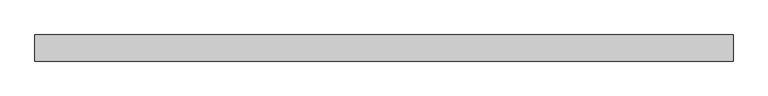
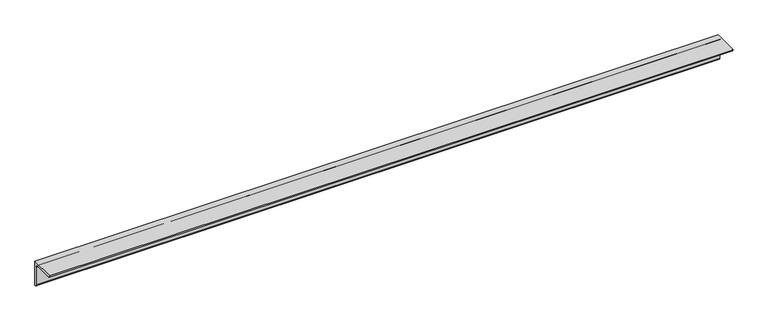
"""IFC4 building model written with IfcOpenShell, lengths in millimetres: member geometry, 0912_Steel Framing_L-KSD3502 : H_SB_AR_S03_L-130x130x12_HBR3."""

from ifc_helpers import new_model, si_unit, point, frame, frame_2d, origin, place, context, project, spatial, polyline, circle_curve, trimmed, segment, composite_curve, outline, extrude, source, transform, mapped, element, save


def member_46ab37a3(model_context):
    return source(origin(), model_context, "Body", "SweptSolid", [
        extrude(outline(composite_curve([segment(polyline([(36.4, 36.4), (36.4, -93.6)]), True, "CONTINUOUS"), segment(trimmed(circle_curve(frame_2d((36.4, -81.6)), 12.0), [point((36.4, -93.6))], [point((24.4, -81.6))], False, "CARTESIAN"), True, "CONTINUOUS"), segment(polyline([(24.4, -81.6), (24.4, 12.4)]), True, "CONTINUOUS"), segment(trimmed(circle_curve(frame_2d((12.4, 12.4)), 12.0), [point((24.4, 12.4))], [point((12.4, 24.4))], True, "CARTESIAN"), True, "CONTINUOUS"), segment(polyline([(12.4, 24.4), (-81.6, 24.4)]), True, "CONTINUOUS"), segment(trimmed(circle_curve(frame_2d((-81.6, 36.4)), 12.0), [point((-81.6, 24.4))], [point((-93.6, 36.4))], False, "CARTESIAN"), True, "CONTINUOUS"), segment(polyline([(-93.6, 36.4), (36.4, 36.4)]), True, "CONTINUOUS")], self_intersect=False)), frame((-1750.5663611, 0.0, 0.0), z_axis=(1.0, 0.0, 0.0), x_axis=(0.0, 1.0, 0.0)), (0.0, 0.0, 1.0), 3476.5545794),
    ])


if __name__ == "__main__":
    model = new_model("IFC4")
    model_context = context("Model", 3, world=origin())
    ifc_project = project(units=[si_unit("LENGTHUNIT", "METRE", prefix="MILLI")], contexts=[model_context])
    site = spatial("IfcSite", under=ifc_project)
    building = spatial("IfcBuilding", under=site)
    placement = place(None, origin())
    member_shape = member_46ab37a3(model_context)
    element("IfcMember", 1, ObjectType="0912_Steel Framing_L-KSD3502 : H_SB_AR_S03_L-130x130x12_HBR3", at=placement, inside=building, context=model_context, shape_type="MappedRepresentation", body=[
        mapped(member_shape, transform((0.0, 0.0, 0.0), x_axis=(1.0, 0.0, 0.0), y_axis=(0.0, 1.0, 0.0), z_axis=(0.0, 0.0, 1.0))),
    ])
    save(model, "model.ifc")

# Revit data of these elements
# Type "0912_Steel Framing_L-KSD3502 : H_SB_AR_S03_L-130x130x12_HBR3"
#   k = 25 mm
#   Perimeter = 0.52 m²/m
#   Nominal Weight = 23.40 kgf/m
#   Length [instance default] = 1000 mm
#   b = 130 mm
#   d = 130 mm
#   t = 12 mm
#   x = 36.4 mm
#   y = 36.4 mm
#   A = 2976.00 m²
#   Structural Material [instance default] = Steel, 45-345
# Element 1 (IfcMember, "0912_Steel Framing_L-KSD3502 : H_SB_AR_S03_L-130x130x12_HBR3")
#   Materials on its faces: "Steel, 45-345"
# Materials
#   "Steel, 45-345": class "Metal", colour RGB 189 187 185, transparency 0, Description = "Steel 345 MPa", Cost = 0
